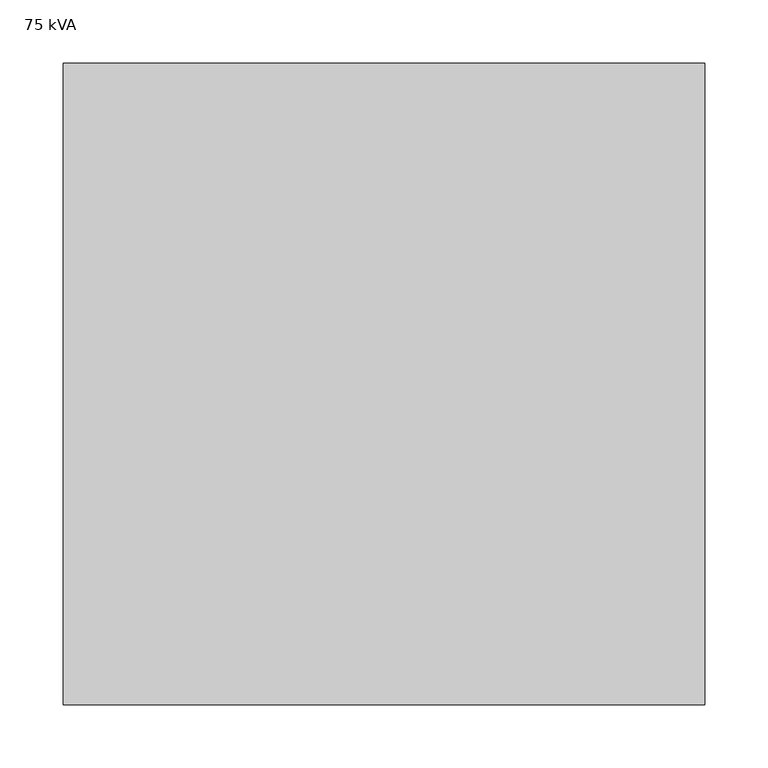
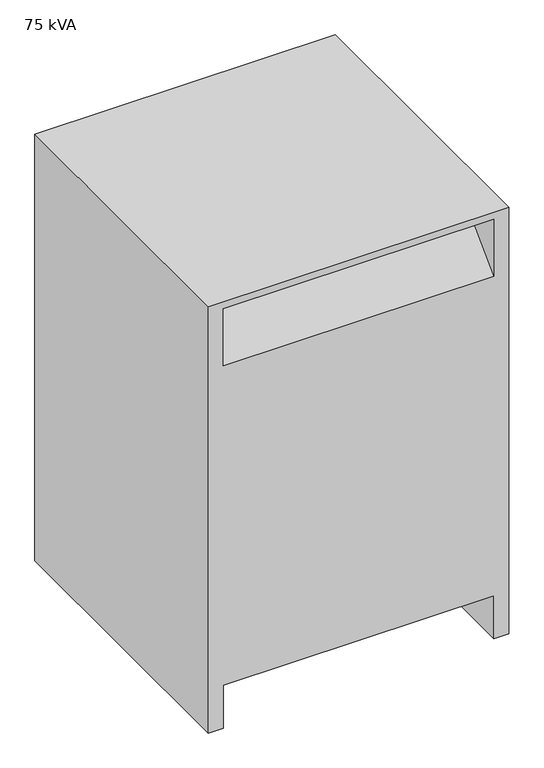
"""IFC4 building model written with IfcOpenShell, lengths in millimetres: proxy geometry, Dry Type Transformer - 480-208Y120 - NEMA Type 2 : 75 kVA."""

import ifcopenshell
import ifcopenshell.guid

model = None  # the IFC model being written
_history = None  # IfcOwnerHistory: only IFC2X3 demands one
_inside = {}  # id of a spatial element -> (the spatial element, [elements in it])
_under = {}  # id of a project, library or spatial element -> (it, [spatial elements below it])
_declared = {}  # id of a project -> (the project, [libraries it declares])
_typed = {}  # id of a type object -> (the type object, [elements of that type])
_made_of = {}  # id of a material, layer set ... -> (it, [elements and type objects made of it])


def new_model(schema):
    """Start an empty IFC model of exactly this schema.

    Asked for "IFC4X3", IfcOpenShell would pick the latest addendum, in which some entities
    have other attributes; the version numbers below select the first issue.
    IFC2X3 requires an IfcOwnerHistory on every rooted entity: one is made here for all.
    """
    global model, _history
    if schema == "IFC4X3":
        model = ifcopenshell.file(schema_version=(4, 3, 0, 0))
    else:
        model = ifcopenshell.file(schema=schema)
    _inside.clear()
    _under.clear()
    _declared.clear()
    _typed.clear()
    _made_of.clear()
    _history = None
    if model.schema == "IFC2X3":
        org = make("IfcOrganization", Name="unknown")
        user = make(
            "IfcPersonAndOrganization",
            ThePerson=make("IfcPerson", FamilyName="unknown"),
            TheOrganization=org,
        )
        app = make(
            "IfcApplication",
            ApplicationDeveloper=org,
            Version="unknown",
            ApplicationFullName="unknown",
            ApplicationIdentifier="unknown",
        )
        _history = make(
            "IfcOwnerHistory",
            OwningUser=user,
            OwningApplication=app,
            ChangeAction="ADDED",
            CreationDate=0,
        )
    return model


def make(cls, **values):
    """One entity of the class cls with the attributes given. An attribute that is None is left unset."""
    return model.create_entity(
        cls, **{name: value for name, value in values.items() if value is not None}
    )


def rooted(cls, **values):
    """An entity with a GlobalId (a new one), such as an element, a storey or a relation."""
    return make(cls, GlobalId=ifcopenshell.guid.new(), OwnerHistory=_history, **values)


def si_unit(unit_type, name, prefix=None):
    """IfcSIUnit, for example si_unit("LENGTHUNIT", "METRE", prefix="MILLI")."""
    return make("IfcSIUnit", UnitType=unit_type, Prefix=prefix, Name=name)


def assignment(units):
    """IfcUnitAssignment: the units of a project."""
    return None if units is None else make("IfcUnitAssignment", Units=units)


def point(xyz):
    """IfcCartesianPoint."""
    return None if xyz is None else make("IfcCartesianPoint", Coordinates=xyz)


def direction(xyz):
    """IfcDirection."""
    return None if xyz is None else make("IfcDirection", DirectionRatios=xyz)


def frame(location, z_axis=None, x_axis=None):
    """IfcAxis2Placement3D, a coordinate frame: its origin and axes. An axis left out is left unset."""
    return make(
        "IfcAxis2Placement3D",
        Location=point(location),
        Axis=direction(z_axis),
        RefDirection=direction(x_axis),
    )


def origin():
    """The frame at (0, 0, 0) with its axes left unset."""
    return frame((0.0, 0.0, 0.0))


def place(relative_to, where):
    """IfcLocalPlacement: puts the frame where relative to a parent placement (None: the world)."""
    return make(
        "IfcLocalPlacement", PlacementRelTo=relative_to, RelativePlacement=where
    )


def context(
    kind, dimensions, precision=None, world=None, true_north=None, identifier=None
):
    """IfcGeometricRepresentationContext, for example the 3D "Model" context."""
    return make(
        "IfcGeometricRepresentationContext",
        ContextIdentifier=identifier,
        ContextType=kind,
        CoordinateSpaceDimension=dimensions,
        Precision=precision,
        WorldCoordinateSystem=world,
        TrueNorth=true_north,
    )


def project(units=None, contexts=None):
    """IfcProject with its units and contexts."""
    return rooted(
        "IfcProject",
        Name="project",
        RepresentationContexts=contexts,
        UnitsInContext=assignment(units),
    )


def spatial(cls, under=None, at=None, **own):
    """A site, building, storey or space (cls), placed at a placement, below another one or the project."""
    s = rooted(cls, ObjectPlacement=at, **own)
    if under is not None:
        _under.setdefault(under.id(), (under, []))[1].append(s)
    return s


def faces_of(points, faces, orient=None, outer=None):
    """IfcFace entities. A face is a list of loops; a loop is a list of indices into points, from 0.

    orient and outer hold one flag for each loop. By default every Orientation is true, the
    first loop of a face is its IfcFaceOuterBound and the others are IfcFaceBound.
    """
    made = []
    for i, loops in enumerate(faces):
        bounds = []
        for j, loop in enumerate(loops):
            is_outer = j == 0 if outer is None else outer[i][j]
            bounds.append(
                make(
                    "IfcFaceOuterBound" if is_outer else "IfcFaceBound",
                    Bound=make("IfcPolyLoop", Polygon=[points[k] for k in loop]),
                    Orientation=True if orient is None else orient[i][j],
                )
            )
        made.append(make("IfcFace", Bounds=bounds))
    return made


def faceted_brep(points, faces, orient=None, outer=None, voids=None):
    """IfcFacetedBrep: a solid bounded by flat faces; with voids (closed shells), ...WithVoids."""
    shared = [point(p) for p in points]
    hull = make("IfcClosedShell", CfsFaces=faces_of(shared, faces, orient, outer))
    if voids is None:
        return make("IfcFacetedBrep", Outer=hull)
    return make(
        "IfcFacetedBrepWithVoids",
        Outer=hull,
        Voids=[
            make(cls, CfsFaces=faces_of(shared, fs, o, b)) for cls, fs, o, b in voids
        ],
    )


def shape(context_of_items, identifier, shape_type, items):
    """IfcShapeRepresentation: the items that make up one representation, for example the "Body"."""
    return make(
        "IfcShapeRepresentation",
        ContextOfItems=context_of_items,
        RepresentationIdentifier=identifier,
        RepresentationType=shape_type,
        Items=items,
    )


def source(mapping_origin, context_of_items, identifier, shape_type, items):
    """IfcRepresentationMap: a shape defined once, which mapped items show again and again."""
    return make(
        "IfcRepresentationMap",
        MappingOrigin=mapping_origin,
        MappedRepresentation=shape(context_of_items, identifier, shape_type, items),
    )


def transform(
    local_origin,
    x_axis=None,
    y_axis=None,
    z_axis=None,
    scale=None,
    scale2=None,
    scale3=None,
    uniform=True,
):
    """IfcCartesianTransformationOperator3D, or its non-uniform kind. x_axis, y_axis, z_axis: its Axis1, 2, 3."""
    if uniform:
        return make(
            "IfcCartesianTransformationOperator3D",
            Axis1=direction(x_axis),
            Axis2=direction(y_axis),
            LocalOrigin=point(local_origin),
            Scale=scale,
            Axis3=direction(z_axis),
        )
    return make(
        "IfcCartesianTransformationOperator3DnonUniform",
        Axis1=direction(x_axis),
        Axis2=direction(y_axis),
        LocalOrigin=point(local_origin),
        Scale=scale,
        Axis3=direction(z_axis),
        Scale2=scale2,
        Scale3=scale3,
    )


def mapped(mapping_source, mapping_target):
    """IfcMappedItem: shows the shape of a source again, moved by a transform."""
    return make(
        "IfcMappedItem", MappingSource=mapping_source, MappingTarget=mapping_target
    )


def made_of(thing, what):
    """Note that an element or type object is made of a material, layer set ...; save() writes the relation."""
    if what is not None:
        _made_of.setdefault(what.id(), (what, []))[1].append(thing)
    return thing


def element(
    cls,
    number,
    at=None,
    inside=None,
    cuts=None,
    type_object=None,
    material=None,
    context=None,
    identifier="Body",
    shape_type=None,
    held_by="IfcProductDefinitionShape",
    body=None,
    shapes=None,
    **own,
):
    """One element of the class cls, such as IfcWall. Its Tag is "e" and its number.

    at: its placement. inside: the storey or other place that contains it. cuts: it is an
    opening in that element (IfcRelVoidsElement). A single representation is given by context,
    identifier, shape_type and body (its items); several are given by shapes. held_by: the class
    of the entity that holds the representations. save() writes the other relations.
    """
    e = rooted(cls, Tag="e%d" % number, ObjectPlacement=at, **own)
    if body is not None:
        shapes = [shape(context, identifier, shape_type, body)]
    if shapes is not None:
        e.Representation = make(held_by, Representations=shapes)
    if inside is not None:
        _inside.setdefault(inside.id(), (inside, []))[1].append(e)
    if cuts is not None:
        rooted(
            "IfcRelVoidsElement", RelatingBuildingElement=cuts, RelatedOpeningElement=e
        )
    if type_object is not None:
        _typed.setdefault(type_object.id(), (type_object, []))[1].append(e)
    return made_of(e, material)


def aggregate(whole, parts):
    """IfcRelAggregates: a whole, such as a stair, and the parts it consists of."""
    return rooted("IfcRelAggregates", RelatingObject=whole, RelatedObjects=parts)


def save(model, path):
    """Write the relations noted so far, then the file.

    IfcRelAggregates (storeys below a building ...), IfcRelContainedInSpatialStructure (elements
    in a storey), IfcRelDefinesByType, IfcRelAssociatesMaterial and IfcRelDeclares: one each for
    every whole, place, type object, material and project.
    """
    for whole, parts in _under.values():
        aggregate(whole, parts)
    for where, things in _inside.values():
        rooted(
            "IfcRelContainedInSpatialStructure",
            RelatedElements=things,
            RelatingStructure=where,
        )
    for kind, things in _typed.values():
        rooted("IfcRelDefinesByType", RelatedObjects=things, RelatingType=kind)
    for what, things in _made_of.values():
        rooted("IfcRelAssociatesMaterial", RelatedObjects=things, RelatingMaterial=what)
    for by, libraries in _declared.values():
        rooted("IfcRelDeclares", RelatingContext=by, RelatedDefinitions=libraries)
    model.write(path)


def proxy_75_kva_f23e4866(model_context):
    return source(origin(), model_context, "Body", "Brep", [
        faceted_brep([(254.0, -123.2841349, 762.0), (254.0, 384.7158651, 762.0), (-254.0, 384.7158651, 762.0), (-254.0, -123.2841349, 762.0), (-254.0, -123.2841349, 0.0), (-254.0, 384.7158651, 0.0), (-228.6, 384.7158651, 0.0), (-228.6, -123.2841349, 0.0), (254.0, 384.7158651, 0.0), (254.0, -123.2841349, 0.0), (228.6, -123.2841349, 0.0), (228.6, 384.7158651, 0.0), (228.6, 384.7158651, 76.2), (-228.6, 384.7158651, 76.2), (228.6, 384.7158651, 647.7), (228.6, 384.7158651, 749.3), (-228.6, 384.7158651, 749.3), (-228.6, 384.7158651, 647.7), (-228.6, -123.2841349, 76.2), (228.6, -123.2841349, 76.2), (228.6, -123.2841349, 749.3), (228.6, -123.2841349, 647.7), (-228.6, -123.2841349, 647.7), (-228.6, -123.2841349, 749.3), (228.6, -21.6841349, 749.3), (-228.6, -21.6841349, 749.3), (228.6, 283.1158651, 749.3), (-228.6, 283.1158651, 749.3)], [[[0, 1, 2, 3]], [[4, 5, 6, 7]], [[8, 9, 10, 11]], [[1, 0, 9, 8]], [[2, 1, 8, 11, 12, 13, 6, 5], [14, 15, 16, 17]], [[3, 2, 5, 4]], [[0, 3, 4, 7, 18, 19, 10, 9], [20, 21, 22, 23]], [[18, 13, 12, 19]], [[13, 18, 7, 6]], [[19, 12, 11, 10]], [[24, 21, 20]], [[25, 23, 22]], [[24, 20, 23, 25]], [[21, 24, 25, 22]], [[26, 15, 14]], [[27, 17, 16]], [[26, 14, 17, 27]], [[15, 26, 27, 16]]]),
    ])


if __name__ == "__main__":
    model = new_model("IFC4")
    model_context = context("Model", 3, world=origin())
    ifc_project = project(units=[si_unit("LENGTHUNIT", "METRE", prefix="MILLI")], contexts=[model_context])
    site = spatial("IfcSite", under=ifc_project)
    building = spatial("IfcBuilding", under=site)
    placement = place(None, origin())
    proxy_75_kva_shape = proxy_75_kva_f23e4866(model_context)
    element("IfcBuildingElementProxy", 1, Name="Dry Type Transformer - 480-208Y120 - NEMA Type 2 : 75 kVA", ObjectType="Dry Type Transformer - 480-208Y120 - NEMA Type 2 : 75 kVA", at=placement, inside=building, context=model_context, shape_type="MappedRepresentation", body=[
        mapped(proxy_75_kva_shape, transform((0.0, 0.0, 0.0), x_axis=(1.0, 0.0, 0.0), y_axis=(0.0, 1.0, 0.0), z_axis=(0.0, 0.0, 1.0))),
    ])
    save(model, "model.ifc")

# Revit data of these elements
# Type "Dry Type Transformer - 480-208Y120 - NEMA Type 2 : 75 kVA"
#   built-in parameter 1140083 [instance default] = "Type 2"
#   Transformer Length = 1' - 8"
#   Primary Voltage = 480 V
#   Transformer Height = 2' - 6"
#   built-in parameter 1140140 [instance default] = 1 (stored number, unit not read)
#   Transformer Width = 1' - 8"
#   built-in parameter 1140142 [instance default] = -1
#   Primary Number of Poles = 3
#   built-in parameter 1140079 [instance default] = 3
#   Transformer Material = none
#   Load Classification = Transformer
#   Default Elevation = 0
#   Assembly Code = ""
#   built-in parameter 1140087 [instance default] = 1
